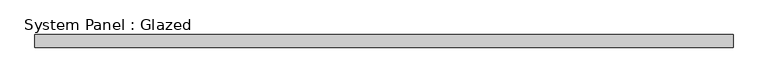
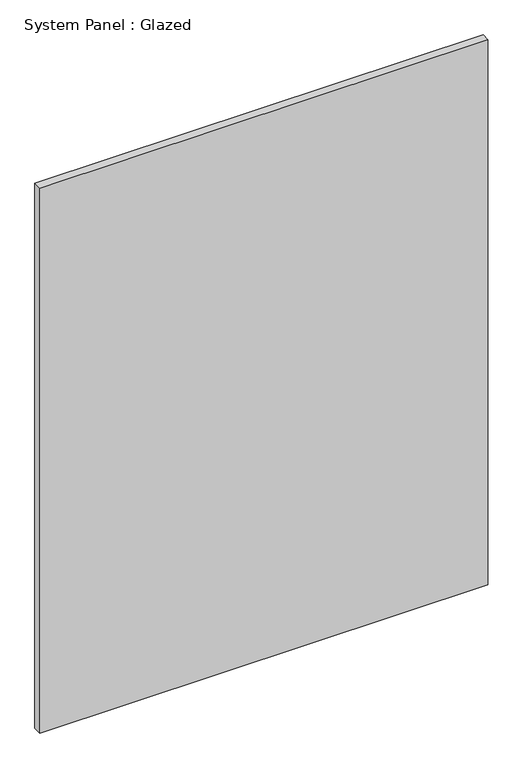
"""IFC4 building model written with IfcOpenShell, lengths in millimetres: plate geometry, System Panel : Glazed."""

from ifc_helpers import new_model, si_unit, origin, origin_with_axes, place, context, project, spatial, polyline, outline, extrude, source, transform, mapped, element, save


def system_panel_glazed_5d43e395(model_context):
    return source(origin(), model_context, "Body", "SweptSolid", [
        extrude(outline(polyline([(669.9999999, 24.5), (-669.9999999, 24.5), (-669.9999999, 49.5), (669.9999999, 49.5), (669.9999999, 24.5)])), origin_with_axes(), (0.0, 0.0, 1.0), 1722.3836314),
    ])


if __name__ == "__main__":
    model = new_model("IFC4")
    model_context = context("Model", 3, world=origin())
    ifc_project = project(units=[si_unit("LENGTHUNIT", "METRE", prefix="MILLI")], contexts=[model_context])
    site = spatial("IfcSite", under=ifc_project)
    building = spatial("IfcBuilding", under=site)
    placement = place(None, origin())
    system_panel_glazed_shape = system_panel_glazed_5d43e395(model_context)
    element("IfcPlate", 1, ObjectType="System Panel : Glazed", at=placement, inside=building, context=model_context, shape_type="MappedRepresentation", body=[
        mapped(system_panel_glazed_shape, transform((0.0, 0.0, 0.0), x_axis=(1.0, 0.0, 0.0), y_axis=(0.0, 1.0, 0.0), z_axis=(0.0, 0.0, 1.0))),
    ])
    save(model, "model.ifc")

# Revit data of these elements
# Element 1 (IfcPlate, "System Panel : Glazed")
#   Materials on its faces: "Glass"
# Materials
#   "Glass": class "Glass", colour RGB 218 227 224, transparency 0.85, Description = "Soda Lime Glass", Cost = 0
